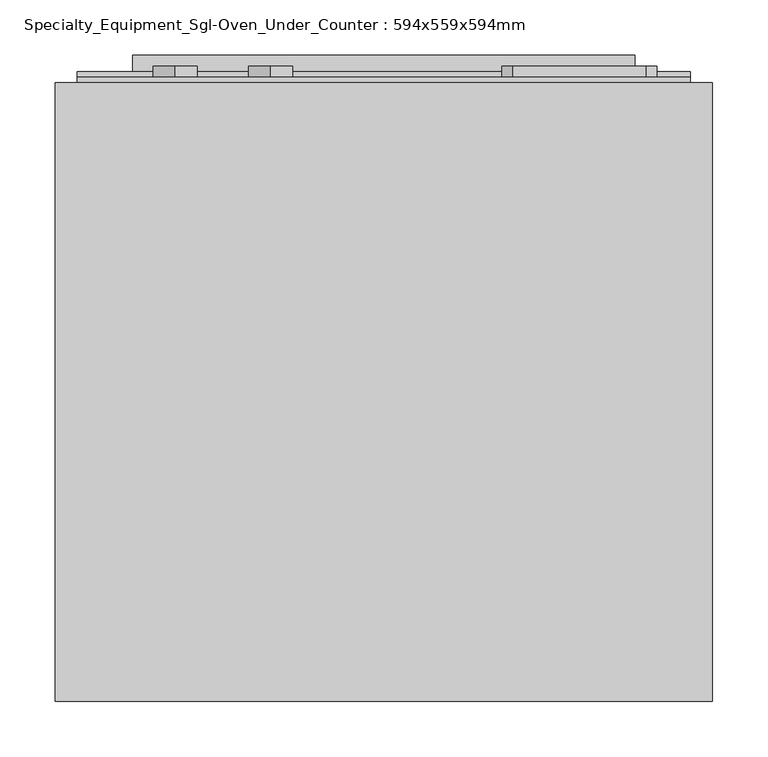
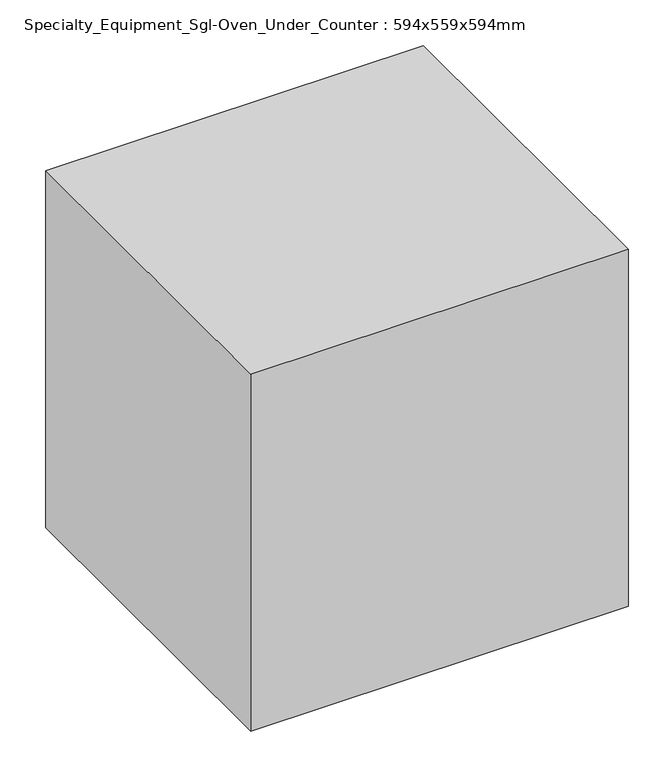
"""IFC4 building model written with IfcOpenShell, lengths in millimetres: proxy geometry, Specialty_Equipment_Sgl-Oven_Under_Counter : 594x559x594mm."""

from ifc_helpers import new_model, si_unit, point, frame, frame_2d, origin, place, context, project, spatial, polyline, circle_curve, trimmed, segment, composite_curve, outline, extrude, faceted_brep, source, transform, mapped, element, save


def specialty_equipment_sgl_oven_under_counter_594x559x594mm_8b8b962d(model_context):
    return source(origin(), model_context, "Body", "SolidModel", [
        faceted_brep([(266.0578446, 665.0, 860.0), (-327.9421554, 665.0, 860.0), (-327.9421554, 106.0, 860.0), (266.0578446, 106.0, 860.0), (266.0578446, 665.0, 266.0), (266.0578446, 106.0, 266.0), (-327.9421554, 106.0, 266.0), (-327.9421554, 665.0, 266.0), (246.0578446, 665.0, 740.4988468), (-307.9421554, 665.0, 740.4988468), (-307.9421554, 665.0, 286.0), (246.0578446, 665.0, 286.0), (246.0578446, 181.9875773, 740.4988468), (246.0578446, 181.9875773, 286.0), (-307.9421554, 181.9875773, 286.0), (-307.9421554, 181.9875773, 740.4988468)], [[[0, 1, 2, 3]], [[4, 5, 6, 7]], [[1, 0, 4, 7], [8, 9, 10, 11]], [[2, 1, 7, 6]], [[3, 2, 6, 5]], [[0, 3, 5, 4]], [[12, 13, 14, 15]], [[12, 15, 9, 8]], [[15, 14, 10, 9]], [[14, 13, 11, 10]], [[13, 12, 8, 11]]]),
        extrude(outline(polyline([(-307.9421554, 670.0), (246.0578446, 670.0), (246.0578446, 665.0), (-307.9421554, 665.0), (-307.9421554, 670.0)])), frame((0.0, 0.0, 740.4988468), z_axis=(0.0, 0.0, 1.0), x_axis=(1.0, 0.0, 0.0)), (0.0, 0.0, 1.0), 99.5011532),
        extrude(outline(polyline([(86.0578446, 680.0), (206.0578446, 680.0), (206.0578446, 665.0), (86.0578446, 665.0), (86.0578446, 680.0)])), frame((0.0, 0.0, 790.4988468), z_axis=(0.0, 0.0, 1.0), x_axis=(1.0, 0.0, 0.0)), (0.0, 0.0, 1.0), 28.8192733),
        extrude(outline(composite_curve([segment(trimmed(circle_curve(frame_2d((785.4988468, -219.501226)), 20.0), [point((805.4988468, -219.501226))], [point((765.4988468, -219.501226))], False, "CARTESIAN"), True, "CONTINUOUS"), segment(trimmed(circle_curve(frame_2d((785.4988468, -219.501226)), 20.0), [point((765.4988468, -219.501226))], [point((805.4988468, -219.501226))], False, "CARTESIAN"), True, "CONTINUOUS")], self_intersect=False)), frame((0.0, 665.0, 0.0), z_axis=(0.0, 1.0, 0.0), x_axis=(0.0, 0.0, 1.0)), (0.0, 0.0, 1.0), 15.0),
        extrude(outline(composite_curve([segment(trimmed(circle_curve(frame_2d((785.4988468, -133.1879639)), 20.0), [point((805.4988468, -133.1879639))], [point((765.4988468, -133.1879639))], False, "CARTESIAN"), True, "CONTINUOUS"), segment(trimmed(circle_curve(frame_2d((785.4988468, -133.1879639)), 20.0), [point((765.4988468, -133.1879639))], [point((805.4988468, -133.1879639))], False, "CARTESIAN"), True, "CONTINUOUS")], self_intersect=False)), frame((0.0, 665.0, 0.0), z_axis=(0.0, 1.0, 0.0), x_axis=(0.0, 0.0, 1.0)), (0.0, 0.0, 1.0), 15.0),
        extrude(outline(composite_curve([segment(trimmed(circle_curve(frame_2d((770.4988468, 86.0578446)), 10.0), [point((780.4988468, 86.0578446))], [point((760.4988468, 86.0578446))], False, "CARTESIAN"), True, "CONTINUOUS"), segment(trimmed(circle_curve(frame_2d((770.4988468, 86.0578446)), 10.0), [point((760.4988468, 86.0578446))], [point((780.4988468, 86.0578446))], False, "CARTESIAN"), True, "CONTINUOUS")], self_intersect=False)), frame((0.0, 665.0, 0.0), z_axis=(0.0, 1.0, 0.0), x_axis=(0.0, 0.0, 1.0)), (0.0, 0.0, 1.0), 15.0),
        extrude(outline(composite_curve([segment(trimmed(circle_curve(frame_2d((770.4988468, 116.0578446)), 10.0), [point((780.4988468, 116.0578446))], [point((760.4988468, 116.0578446))], False, "CARTESIAN"), True, "CONTINUOUS"), segment(trimmed(circle_curve(frame_2d((770.4988468, 116.0578446)), 10.0), [point((760.4988468, 116.0578446))], [point((780.4988468, 116.0578446))], False, "CARTESIAN"), True, "CONTINUOUS")], self_intersect=False)), frame((0.0, 665.0, 0.0), z_axis=(0.0, 1.0, 0.0), x_axis=(0.0, 0.0, 1.0)), (0.0, 0.0, 1.0), 15.0),
        extrude(outline(composite_curve([segment(trimmed(circle_curve(frame_2d((770.4988468, 146.0578446)), 10.0), [point((780.4988468, 146.0578446))], [point((760.4988468, 146.0578446))], False, "CARTESIAN"), True, "CONTINUOUS"), segment(trimmed(circle_curve(frame_2d((770.4988468, 146.0578446)), 10.0), [point((760.4988468, 146.0578446))], [point((780.4988468, 146.0578446))], False, "CARTESIAN"), True, "CONTINUOUS")], self_intersect=False)), frame((0.0, 665.0, 0.0), z_axis=(0.0, 1.0, 0.0), x_axis=(0.0, 0.0, 1.0)), (0.0, 0.0, 1.0), 15.0),
        extrude(outline(composite_curve([segment(trimmed(circle_curve(frame_2d((770.4988468, 176.0578446)), 10.0), [point((780.4988468, 176.0578446))], [point((760.4988468, 176.0578446))], False, "CARTESIAN"), True, "CONTINUOUS"), segment(trimmed(circle_curve(frame_2d((770.4988468, 176.0578446)), 10.0), [point((760.4988468, 176.0578446))], [point((780.4988468, 176.0578446))], False, "CARTESIAN"), True, "CONTINUOUS")], self_intersect=False)), frame((0.0, 665.0, 0.0), z_axis=(0.0, 1.0, 0.0), x_axis=(0.0, 0.0, 1.0)), (0.0, 0.0, 1.0), 15.0),
        extrude(outline(composite_curve([segment(trimmed(circle_curve(frame_2d((770.4988468, 206.0578446)), 10.0), [point((780.4988468, 206.0578446))], [point((760.4988468, 206.0578446))], False, "CARTESIAN"), True, "CONTINUOUS"), segment(trimmed(circle_curve(frame_2d((770.4988468, 206.0578446)), 10.0), [point((760.4988468, 206.0578446))], [point((780.4988468, 206.0578446))], False, "CARTESIAN"), True, "CONTINUOUS")], self_intersect=False)), frame((0.0, 665.0, 0.0), z_axis=(0.0, 1.0, 0.0), x_axis=(0.0, 0.0, 1.0)), (0.0, 0.0, 1.0), 15.0),
        extrude(outline(polyline([(-257.9421554, 690.0), (196.0578446, 690.0), (196.0578446, 675.0), (-257.9421554, 675.0), (-257.9421554, 690.0)])), frame((0.0, 0.0, 697.6588468), z_axis=(0.0, 0.0, 1.0), x_axis=(1.0, 0.0, 0.0)), (0.0, 0.0, 1.0), 20.0),
        extrude(outline(polyline([(286.0, -307.9421554), (286.0, 246.0578446), (740.4988468, 246.0578446), (740.4988468, -307.9421554), (286.0, -307.9421554)]), holes=[polyline([(336.0, -267.9421554), (667.6588468, -267.9421554), (667.6588468, 206.0578446), (336.0, 206.0578446), (336.0, -267.9421554)])]), frame((0.0, 665.0, 0.0), z_axis=(0.0, 1.0, 0.0), x_axis=(0.0, 0.0, 1.0)), (0.0, 0.0, 1.0), 10.0),
    ])


if __name__ == "__main__":
    model = new_model("IFC4")
    model_context = context("Model", 3, world=origin())
    ifc_project = project(units=[si_unit("LENGTHUNIT", "METRE", prefix="MILLI")], contexts=[model_context])
    site = spatial("IfcSite", under=ifc_project)
    building = spatial("IfcBuilding", under=site)
    placement = place(None, origin())
    specialty_equipment_sgl_oven_under_counter_594x559x594mm_shape = specialty_equipment_sgl_oven_under_counter_594x559x594mm_8b8b962d(model_context)
    element("IfcBuildingElementProxy", 1, Name="Specialty_Equipment_Sgl-Oven_Under_Counter : 594x559x594mm", ObjectType="Specialty_Equipment_Sgl-Oven_Under_Counter : 594x559x594mm", at=placement, inside=building, context=model_context, shape_type="MappedRepresentation", body=[
        mapped(specialty_equipment_sgl_oven_under_counter_594x559x594mm_shape, transform((0.0, 0.0, 0.0), x_axis=(1.0, 0.0, 0.0), y_axis=(0.0, 1.0, 0.0), z_axis=(0.0, 0.0, 1.0))),
    ])
    save(model, "model.ifc")

# Revit data of these elements
# Type "Specialty_Equipment_Sgl-Oven_Under_Counter : 594x559x594mm"
#   Label = "OVEN"
#   Keynote = "N"
#   Depth = 559 mm
#   Height = 594 mm
#   Placement Hgt = 266 mm
#   Width = 594 mm
#   Oven Material = Metal - Stainless Steel
# Element 1 (IfcBuildingElementProxy, "Specialty_Equipment_Sgl-Oven_Under_Counter : 594x559x594mm")
#   Materials on its faces: "Metal - Paint Finish - Dark Gray, Matte", "Metal - Stainless Steel", "Plastic - Black"
# Materials
#   "Metal - Stainless Steel": class "Metal", colour RGB 173 173 173, transparency 0
#   "Metal - Paint Finish - Dark Gray, Matte": class "Paint", colour RGB 98 98 98, transparency 0
#   "Plastic - Black": class "Plastic", colour RGB 0 0 0, transparency 0
